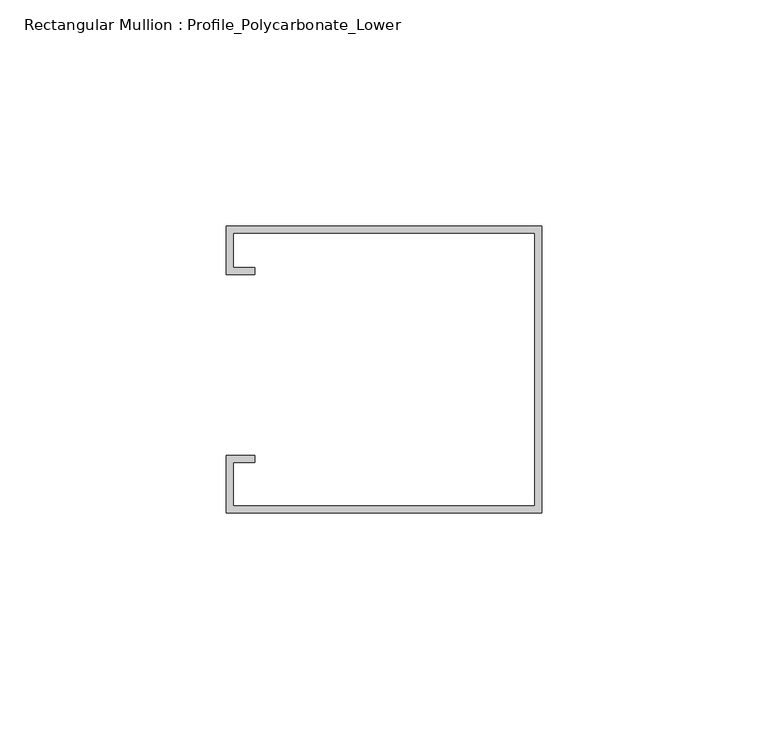
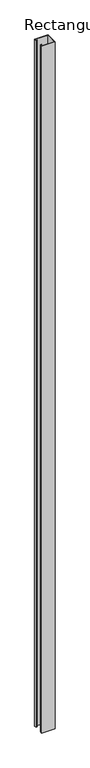
"""IFC4 building model written with IfcOpenShell, lengths in millimetres: member geometry, Rectangular Mullion : Profile_Polycarbonate_Lower."""

from ifc_helpers import new_model, si_unit, frame, origin, place, context, project, spatial, polyline, outline, extrude, source, transform, mapped, element, save


def rectangular_mullion_profile_polycarbonate_lower_69692f3e(model_context):
    return source(origin(), model_context, "Body", "SweptSolid", [
        extrude(outline(polyline([(0.0, -32.7), (-69.85, -32.7), (-69.85, -20.0), (-63.5, -20.0), (-63.5, -21.5875), (-68.2625, -21.5875), (-68.2625, -31.1125), (-1.5875, -31.1125), (-1.5875, 29.2125), (-68.2625, 29.2125), (-68.2625, 21.5875), (-63.5, 21.5875), (-63.5, 20.0), (-69.85, 20.0), (-69.85, 30.8), (0.0, 30.8), (0.0, -32.7)])), frame((0.0, 0.0, -3807.775), z_axis=(0.0, 0.0, 1.0), x_axis=(1.0, 0.0, 0.0)), (0.0, 0.0, 1.0), 3807.775),
    ])


if __name__ == "__main__":
    model = new_model("IFC4")
    model_context = context("Model", 3, world=origin())
    ifc_project = project(units=[si_unit("LENGTHUNIT", "METRE", prefix="MILLI")], contexts=[model_context])
    site = spatial("IfcSite", under=ifc_project)
    building = spatial("IfcBuilding", under=site)
    placement = place(None, origin())
    rectangular_mullion_profile_polycarbonate_lower_shape = rectangular_mullion_profile_polycarbonate_lower_69692f3e(model_context)
    element("IfcMember", 1, ObjectType="Rectangular Mullion : Profile_Polycarbonate_Lower", at=placement, inside=building, context=model_context, shape_type="MappedRepresentation", body=[
        mapped(rectangular_mullion_profile_polycarbonate_lower_shape, transform((0.0, 0.0, 0.0), x_axis=(1.0, 0.0, 0.0), y_axis=(0.0, 1.0, 0.0), z_axis=(0.0, 0.0, 1.0))),
    ])
    save(model, "model.ifc")

# Revit data of these elements
# Type "Rectangular Mullion : Profile_Polycarbonate_Lower"
#   built-in parameter 1007322 = 0.208333 (stored number, unit not read)
#   built-in parameter 1007321 = 0 (stored number, unit not read)
#   built-in parameter 1007320 = 0.00520833 (stored number, unit not read)
# Element 1 (IfcMember, "Rectangular Mullion : Profile_Polycarbonate_Lower")
#   Materials on its faces: "ALUMINUM PROFILE AT POLYCARBONATE PANEL"
# Materials
#   "ALUMINUM PROFILE AT POLYCARBONATE PANEL": class "Metal", colour RGB 244 244 244, transparency 0, Description = "Aluminum 6061", Cost = 0
